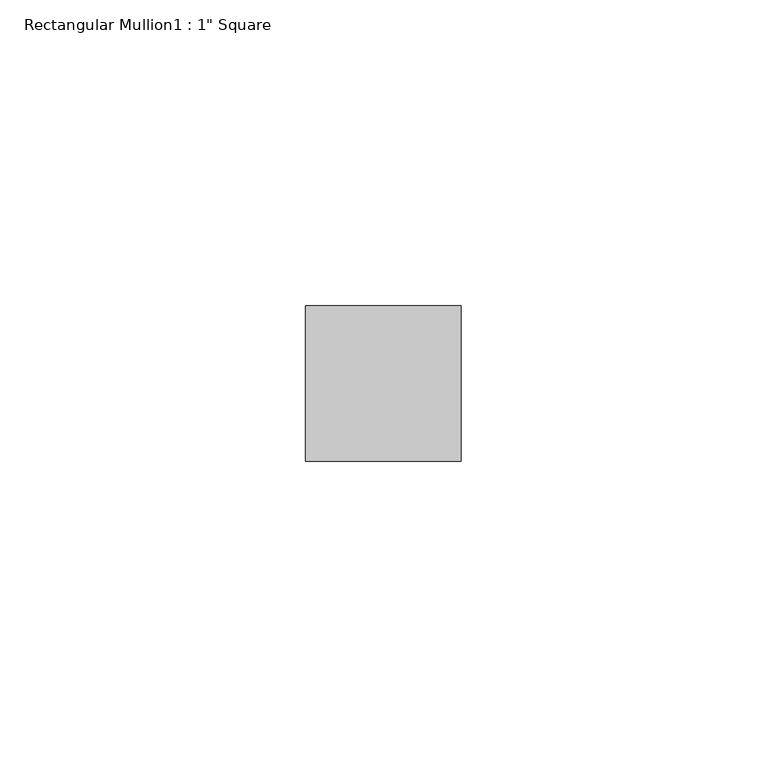
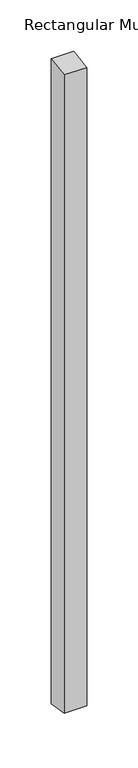
"""IFC4 building model written with IfcOpenShell, lengths in millimetres: member geometry."""

import ifcopenshell
import ifcopenshell.guid

model = None  # the IFC model being written
_history = None  # IfcOwnerHistory: only IFC2X3 demands one
_inside = {}  # id of a spatial element -> (the spatial element, [elements in it])
_under = {}  # id of a project, library or spatial element -> (it, [spatial elements below it])
_declared = {}  # id of a project -> (the project, [libraries it declares])
_typed = {}  # id of a type object -> (the type object, [elements of that type])
_made_of = {}  # id of a material, layer set ... -> (it, [elements and type objects made of it])


def new_model(schema):
    """Start an empty IFC model of exactly this schema.

    Asked for "IFC4X3", IfcOpenShell would pick the latest addendum, in which some entities
    have other attributes; the version numbers below select the first issue.
    IFC2X3 requires an IfcOwnerHistory on every rooted entity: one is made here for all.
    """
    global model, _history
    if schema == "IFC4X3":
        model = ifcopenshell.file(schema_version=(4, 3, 0, 0))
    else:
        model = ifcopenshell.file(schema=schema)
    _inside.clear()
    _under.clear()
    _declared.clear()
    _typed.clear()
    _made_of.clear()
    _history = None
    if model.schema == "IFC2X3":
        org = make("IfcOrganization", Name="unknown")
        user = make(
            "IfcPersonAndOrganization",
            ThePerson=make("IfcPerson", FamilyName="unknown"),
            TheOrganization=org,
        )
        app = make(
            "IfcApplication",
            ApplicationDeveloper=org,
            Version="unknown",
            ApplicationFullName="unknown",
            ApplicationIdentifier="unknown",
        )
        _history = make(
            "IfcOwnerHistory",
            OwningUser=user,
            OwningApplication=app,
            ChangeAction="ADDED",
            CreationDate=0,
        )
    return model


def make(cls, **values):
    """One entity of the class cls with the attributes given. An attribute that is None is left unset."""
    return model.create_entity(
        cls, **{name: value for name, value in values.items() if value is not None}
    )


def rooted(cls, **values):
    """An entity with a GlobalId (a new one), such as an element, a storey or a relation."""
    return make(cls, GlobalId=ifcopenshell.guid.new(), OwnerHistory=_history, **values)


def si_unit(unit_type, name, prefix=None):
    """IfcSIUnit, for example si_unit("LENGTHUNIT", "METRE", prefix="MILLI")."""
    return make("IfcSIUnit", UnitType=unit_type, Prefix=prefix, Name=name)


def assignment(units):
    """IfcUnitAssignment: the units of a project."""
    return None if units is None else make("IfcUnitAssignment", Units=units)


def point(xyz):
    """IfcCartesianPoint."""
    return None if xyz is None else make("IfcCartesianPoint", Coordinates=xyz)


def direction(xyz):
    """IfcDirection."""
    return None if xyz is None else make("IfcDirection", DirectionRatios=xyz)


def frame(location, z_axis=None, x_axis=None):
    """IfcAxis2Placement3D, a coordinate frame: its origin and axes. An axis left out is left unset."""
    return make(
        "IfcAxis2Placement3D",
        Location=point(location),
        Axis=direction(z_axis),
        RefDirection=direction(x_axis),
    )


def origin():
    """The frame at (0, 0, 0) with its axes left unset."""
    return frame((0.0, 0.0, 0.0))


def place(relative_to, where):
    """IfcLocalPlacement: puts the frame where relative to a parent placement (None: the world)."""
    return make(
        "IfcLocalPlacement", PlacementRelTo=relative_to, RelativePlacement=where
    )


def context(
    kind, dimensions, precision=None, world=None, true_north=None, identifier=None
):
    """IfcGeometricRepresentationContext, for example the 3D "Model" context."""
    return make(
        "IfcGeometricRepresentationContext",
        ContextIdentifier=identifier,
        ContextType=kind,
        CoordinateSpaceDimension=dimensions,
        Precision=precision,
        WorldCoordinateSystem=world,
        TrueNorth=true_north,
    )


def project(units=None, contexts=None):
    """IfcProject with its units and contexts."""
    return rooted(
        "IfcProject",
        Name="project",
        RepresentationContexts=contexts,
        UnitsInContext=assignment(units),
    )


def spatial(cls, under=None, at=None, **own):
    """A site, building, storey or space (cls), placed at a placement, below another one or the project."""
    s = rooted(cls, ObjectPlacement=at, **own)
    if under is not None:
        _under.setdefault(under.id(), (under, []))[1].append(s)
    return s


def polyline(points):
    """IfcPolyline through the points."""
    return make("IfcPolyline", Points=[point(p) for p in points])


def outline(outer, holes=None, kind="AREA"):
    """IfcArbitraryClosedProfileDef: a profile drawn as a closed curve; with holes, ...WithVoids."""
    if holes is None:
        return make("IfcArbitraryClosedProfileDef", ProfileType=kind, OuterCurve=outer)
    return make(
        "IfcArbitraryProfileDefWithVoids",
        ProfileType=kind,
        OuterCurve=outer,
        InnerCurves=holes,
    )


def extrude(swept, where, along, depth):
    """IfcExtrudedAreaSolid: the profile swept, set in the frame where, extruded along a direction by depth."""
    return make(
        "IfcExtrudedAreaSolid",
        SweptArea=swept,
        Position=where,
        ExtrudedDirection=direction(along),
        Depth=depth,
    )


def shape(context_of_items, identifier, shape_type, items):
    """IfcShapeRepresentation: the items that make up one representation, for example the "Body"."""
    return make(
        "IfcShapeRepresentation",
        ContextOfItems=context_of_items,
        RepresentationIdentifier=identifier,
        RepresentationType=shape_type,
        Items=items,
    )


def source(mapping_origin, context_of_items, identifier, shape_type, items):
    """IfcRepresentationMap: a shape defined once, which mapped items show again and again."""
    return make(
        "IfcRepresentationMap",
        MappingOrigin=mapping_origin,
        MappedRepresentation=shape(context_of_items, identifier, shape_type, items),
    )


def transform(
    local_origin,
    x_axis=None,
    y_axis=None,
    z_axis=None,
    scale=None,
    scale2=None,
    scale3=None,
    uniform=True,
):
    """IfcCartesianTransformationOperator3D, or its non-uniform kind. x_axis, y_axis, z_axis: its Axis1, 2, 3."""
    if uniform:
        return make(
            "IfcCartesianTransformationOperator3D",
            Axis1=direction(x_axis),
            Axis2=direction(y_axis),
            LocalOrigin=point(local_origin),
            Scale=scale,
            Axis3=direction(z_axis),
        )
    return make(
        "IfcCartesianTransformationOperator3DnonUniform",
        Axis1=direction(x_axis),
        Axis2=direction(y_axis),
        LocalOrigin=point(local_origin),
        Scale=scale,
        Axis3=direction(z_axis),
        Scale2=scale2,
        Scale3=scale3,
    )


def mapped(mapping_source, mapping_target):
    """IfcMappedItem: shows the shape of a source again, moved by a transform."""
    return make(
        "IfcMappedItem", MappingSource=mapping_source, MappingTarget=mapping_target
    )


def made_of(thing, what):
    """Note that an element or type object is made of a material, layer set ...; save() writes the relation."""
    if what is not None:
        _made_of.setdefault(what.id(), (what, []))[1].append(thing)
    return thing


def element(
    cls,
    number,
    at=None,
    inside=None,
    cuts=None,
    type_object=None,
    material=None,
    context=None,
    identifier="Body",
    shape_type=None,
    held_by="IfcProductDefinitionShape",
    body=None,
    shapes=None,
    **own,
):
    """One element of the class cls, such as IfcWall. Its Tag is "e" and its number.

    at: its placement. inside: the storey or other place that contains it. cuts: it is an
    opening in that element (IfcRelVoidsElement). A single representation is given by context,
    identifier, shape_type and body (its items); several are given by shapes. held_by: the class
    of the entity that holds the representations. save() writes the other relations.
    """
    e = rooted(cls, Tag="e%d" % number, ObjectPlacement=at, **own)
    if body is not None:
        shapes = [shape(context, identifier, shape_type, body)]
    if shapes is not None:
        e.Representation = make(held_by, Representations=shapes)
    if inside is not None:
        _inside.setdefault(inside.id(), (inside, []))[1].append(e)
    if cuts is not None:
        rooted(
            "IfcRelVoidsElement", RelatingBuildingElement=cuts, RelatedOpeningElement=e
        )
    if type_object is not None:
        _typed.setdefault(type_object.id(), (type_object, []))[1].append(e)
    return made_of(e, material)


def aggregate(whole, parts):
    """IfcRelAggregates: a whole, such as a stair, and the parts it consists of."""
    return rooted("IfcRelAggregates", RelatingObject=whole, RelatedObjects=parts)


def save(model, path):
    """Write the relations noted so far, then the file.

    IfcRelAggregates (storeys below a building ...), IfcRelContainedInSpatialStructure (elements
    in a storey), IfcRelDefinesByType, IfcRelAssociatesMaterial and IfcRelDeclares: one each for
    every whole, place, type object, material and project.
    """
    for whole, parts in _under.values():
        aggregate(whole, parts)
    for where, things in _inside.values():
        rooted(
            "IfcRelContainedInSpatialStructure",
            RelatedElements=things,
            RelatingStructure=where,
        )
    for kind, things in _typed.values():
        rooted("IfcRelDefinesByType", RelatedObjects=things, RelatingType=kind)
    for what, things in _made_of.values():
        rooted("IfcRelAssociatesMaterial", RelatedObjects=things, RelatingMaterial=what)
    for by, libraries in _declared.values():
        rooted("IfcRelDeclares", RelatingContext=by, RelatedDefinitions=libraries)
    model.write(path)


def member_4057df82(model_context):
    return source(origin(), model_context, "Body", "SweptSolid", [
        extrude(outline(polyline([(-44.45, -7.0452458), (-19.05, -3.019391), (-19.05, -772.1183016), (-44.45, -768.0924469), (-44.45, -7.0452458)])), frame((-12.7, 0.0, 0.0), z_axis=(1.0, 0.0, 0.0), x_axis=(0.0, 1.0, 0.0)), (0.0, 0.0, 1.0), 25.4),
    ])


if __name__ == "__main__":
    model = new_model("IFC4")
    model_context = context("Model", 3, world=origin())
    ifc_project = project(units=[si_unit("LENGTHUNIT", "METRE", prefix="MILLI")], contexts=[model_context])
    site = spatial("IfcSite", under=ifc_project)
    building = spatial("IfcBuilding", under=site)
    placement = place(None, origin())
    member_shape = member_4057df82(model_context)
    element("IfcMember", 1, ObjectType="Rectangular Mullion1 : 1\" Square", at=placement, inside=building, context=model_context, shape_type="MappedRepresentation", body=[
        mapped(member_shape, transform((0.0, 0.0, 0.0), x_axis=(1.0, 0.0, 0.0), y_axis=(0.0, 1.0, 0.0), z_axis=(0.0, 0.0, 1.0))),
    ])
    save(model, "model.ifc")

# Revit data of these elements
# Type "Rectangular Mullion1 : 1\" Square"
#   built-in parameter 1007351 = 0.104167 (stored number, unit not read)
#   built-in parameter 1007304 = 0.0833333 (stored number, unit not read)
#   built-in parameter 1007301 = 0.0416667 (stored number, unit not read)
#   built-in parameter 1007300 = 0.0416667 (stored number, unit not read)
